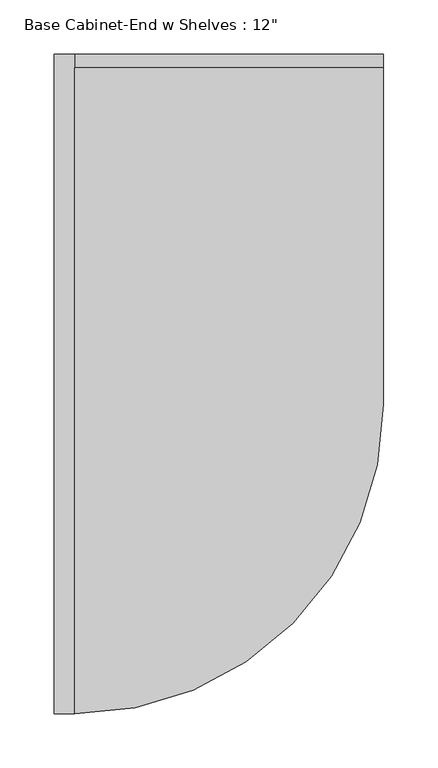
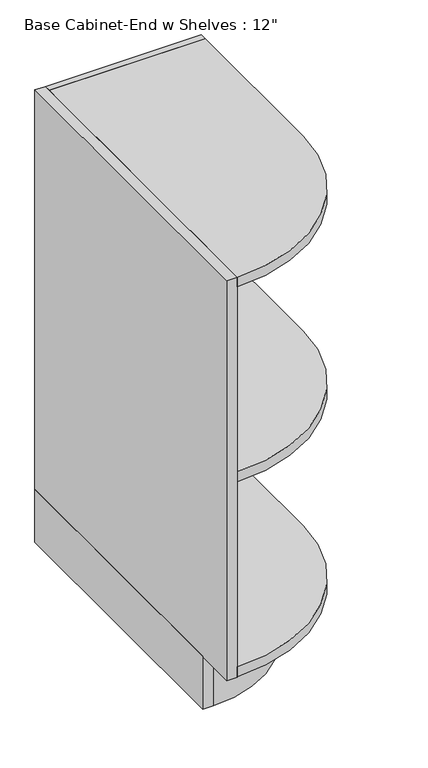
"""IFC4 building model written with IfcOpenShell, lengths in millimetres: furniture geometry."""

from ifc_helpers import new_model, si_unit, point, frame, frame_2d, origin, origin_with_axes, place, context, project, spatial, polyline, circle_curve, trimmed, segment, composite_curve, outline, extrude, source, transform, mapped, element, save


def furniture_b5875d2f(model_context):
    return source(origin(), model_context, "Body", "SweptSolid", [
        extrude(outline(composite_curve([segment(polyline([(228.6, 0.0), (228.6, -323.8500002)]), True, "CONTINUOUS"), segment(trimmed(circle_curve(frame_2d((19.0500002, -323.8500002)), 209.5499998), [point((228.6, -323.8500002))], [point((19.0500002, -533.4))], False, "CARTESIAN"), True, "CONTINUOUS"), segment(polyline([(19.0500002, -533.4), (0.0, -533.4), (0.0, 0.0), (228.6, 0.0)]), True, "CONTINUOUS")], self_intersect=False)), origin_with_axes(), (0.0, 0.0, 1.0), 102.790625),
        extrude(outline(composite_curve([segment(polyline([(304.8, -12.7), (304.8, -323.8499999)]), True, "CONTINUOUS"), segment(trimmed(circle_curve(frame_2d((19.05, -323.8499999)), 285.75), [point((304.8, -323.8499999))], [point((19.05, -609.5999998))], False, "CARTESIAN"), True, "CONTINUOUS"), segment(polyline([(19.05, -609.5999998), (19.05, -12.7), (304.8, -12.7)]), True, "CONTINUOUS")], self_intersect=False)), frame((0.0, 0.0, 102.790625), z_axis=(0.0, 0.0, 1.0), x_axis=(1.0, 0.0, 0.0)), (0.0, 0.0, 1.0), 19.05),
        extrude(outline(composite_curve([segment(polyline([(19.05, -12.7), (304.8, -12.7), (304.8, -323.85)]), True, "CONTINUOUS"), segment(trimmed(circle_curve(frame_2d((19.05, -323.85)), 285.75), [point((304.8, -323.85))], [point((19.05, -609.6))], False, "CARTESIAN"), True, "CONTINUOUS"), segment(polyline([(19.05, -609.6), (19.05, -12.7)]), True, "CONTINUOUS")], self_intersect=False)), frame((0.0, 0.0, 858.440625), z_axis=(0.0, 0.0, 1.0), x_axis=(1.0, 0.0, 0.0)), (0.0, 0.0, 1.0), 19.05),
        extrude(outline(polyline([(0.0, 0.0), (19.05, 0.0), (19.05, -609.6), (0.0, -609.6), (0.0, 0.0)])), frame((0.0, 0.0, 101.6), z_axis=(0.0, 0.0, 1.0), x_axis=(1.0, 0.0, 0.0)), (0.0, 0.0, 1.0), 775.890625),
        extrude(outline(polyline([(304.8, 0.0), (304.8, -12.7), (19.05, -12.7), (19.05, 0.0), (304.8, 0.0)])), frame((0.0, 0.0, 101.6), z_axis=(0.0, 0.0, 1.0), x_axis=(1.0, 0.0, 0.0)), (0.0, 0.0, 1.0), 775.890625),
        extrude(outline(composite_curve([segment(polyline([(304.8, -12.7), (304.8, -323.85)]), True, "CONTINUOUS"), segment(trimmed(circle_curve(frame_2d((19.05, -323.85)), 285.75), [point((304.8, -323.85))], [point((19.05, -609.6))], False, "CARTESIAN"), True, "CONTINUOUS"), segment(polyline([(19.05, -609.6), (19.05, -12.7), (304.8, -12.7)]), True, "CONTINUOUS")], self_intersect=False)), frame((0.0, 0.0, 480.615625), z_axis=(0.0, 0.0, 1.0), x_axis=(1.0, 0.0, 0.0)), (0.0, 0.0, 1.0), 19.05),
    ])


if __name__ == "__main__":
    model = new_model("IFC4")
    model_context = context("Model", 3, world=origin())
    ifc_project = project(units=[si_unit("LENGTHUNIT", "METRE", prefix="MILLI")], contexts=[model_context])
    site = spatial("IfcSite", under=ifc_project)
    building = spatial("IfcBuilding", under=site)
    placement = place(None, origin())
    furniture_shape = furniture_b5875d2f(model_context)
    element("IfcFurniture", 1, ObjectType="Base Cabinet-End w Shelves : 12\"", at=placement, inside=building, context=model_context, shape_type="MappedRepresentation", body=[
        mapped(furniture_shape, transform((0.0, 0.0, 0.0), x_axis=(1.0, 0.0, 0.0), y_axis=(0.0, 1.0, 0.0), z_axis=(0.0, 0.0, 1.0))),
    ])
    save(model, "model.ifc")

# Revit data of these elements
# Type "Base Cabinet-End w Shelves : 12\""
#   COBie.Type.CreatedBy = "doug.wood@us.ibm.com"
#   COBie.Type.CreatedOn = "2016-04-14T02:14:45"
#   COBie.Type.Name = "Casework_Base Cabinet-End w Shelves_12\""
#   COBie.Type.Category = "C1030410"
#   COBie.Type.Description = "Base Cabinet-End w Shelves_12\""
#   COBie.Type.Manufacturer = ""
#   COBie.Type.ModelNumber = ""
#   Assembly Code = "C1030410"
#   COBie.Type.ReplacementCost = 0
#   Width = 1' - 0"
#   Toe Kick Depth = 0' - 3"
#   Height = 2' - 10 1/2"
#   Depth = 2' - 0"
#   COBie.Type = no
#   Cabinet Material = Cabinets
# Element 1 (IfcFurniture, "Base Cabinet-End w Shelves : 12\"")
#   Materials on its faces: "Cabinets"
# Materials
#   "Cabinets": class "Miscellaneous", colour RGB 249 249 249, transparency 0
